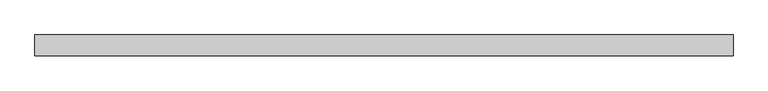
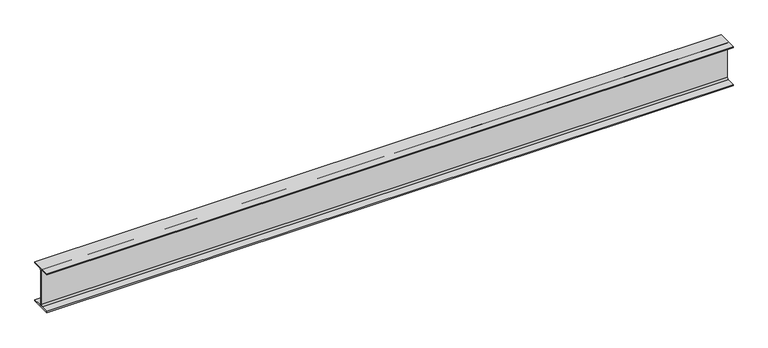
"""IFC4 building model written with IfcOpenShell, lengths in millimetres: beam geometry, 0912_Steel Framing_H-KSD3502 : H_SB_ASB_H-350x175x7x11."""

from ifc_helpers import new_model, si_unit, point, frame, frame_2d, origin, place, context, project, spatial, polyline, circle_curve, trimmed, segment, composite_curve, outline, extrude, source, transform, mapped, element, save


def beam_dbd466da(model_context):
    return source(origin(), model_context, "Body", "SweptSolid", [
        extrude(outline(composite_curve([segment(polyline([(87.5, -164.0), (87.5, -175.0), (-87.5, -175.0), (-87.5, -164.0), (-17.5, -164.0)]), True, "CONTINUOUS"), segment(trimmed(circle_curve(frame_2d((-17.5, -150.0)), 14.0), [point((-17.5, -164.0))], [point((-3.5, -150.0))], True, "CARTESIAN"), True, "CONTINUOUS"), segment(polyline([(-3.5, -150.0), (-3.5, 150.0)]), True, "CONTINUOUS"), segment(trimmed(circle_curve(frame_2d((-17.5, 150.0)), 14.0), [point((-3.5, 150.0))], [point((-17.5, 164.0))], True, "CARTESIAN"), True, "CONTINUOUS"), segment(polyline([(-17.5, 164.0), (-87.5, 164.0), (-87.5, 175.0), (87.5, 175.0), (87.5, 164.0), (17.5, 164.0)]), True, "CONTINUOUS"), segment(trimmed(circle_curve(frame_2d((17.5, 150.0)), 14.0), [point((17.5, 164.0))], [point((3.5, 150.0))], True, "CARTESIAN"), True, "CONTINUOUS"), segment(polyline([(3.5, 150.0), (3.5, -150.0)]), True, "CONTINUOUS"), segment(trimmed(circle_curve(frame_2d((17.5, -150.0)), 14.0), [point((3.5, -150.0))], [point((17.5, -164.0))], True, "CARTESIAN"), True, "CONTINUOUS"), segment(polyline([(17.5, -164.0), (87.5, -164.0)]), True, "CONTINUOUS")], self_intersect=False)), frame((-2912.1972294, 0.0, 0.0), z_axis=(1.0, 0.0, 0.0), x_axis=(0.0, 1.0, 0.0)), (0.0, 0.0, 1.0), 5810.2298939),
    ])


if __name__ == "__main__":
    model = new_model("IFC4")
    model_context = context("Model", 3, world=origin())
    ifc_project = project(units=[si_unit("LENGTHUNIT", "METRE", prefix="MILLI")], contexts=[model_context])
    site = spatial("IfcSite", under=ifc_project)
    building = spatial("IfcBuilding", under=site)
    placement = place(None, origin())
    beam_shape = beam_dbd466da(model_context)
    element("IfcBeam", 1, ObjectType="0912_Steel Framing_H-KSD3502 : H_SB_ASB_H-350x175x7x11", at=placement, inside=building, context=model_context, shape_type="MappedRepresentation", body=[
        mapped(beam_shape, transform((0.0, 0.0, 0.0), x_axis=(1.0, 0.0, 0.0), y_axis=(0.0, 1.0, 0.0), z_axis=(0.0, 0.0, 1.0))),
    ])
    save(model, "model.ifc")

# Revit data of these elements
# Type "0912_Steel Framing_H-KSD3502 : H_SB_ASB_H-350x175x7x11"
#   H_WM Code_1 = "S01AA002-00001 | Main Steel Structure Fabrication Work | Shelter/Building | Medium Steel - Standard (90KG/M>Weight≥30KG/M) | Material: (   )"
#   H_WM Code_2 = "S03AA028-00001 | Main Steel Structure Erection Work | Shelter/Building | Medium Steel (90KG/M>Weight≥30KG/M) | Material: (   )"
#   H_WM Code_3 = "S01AA010-00001 | Main Steel Structure Fabrication Work | Shelter/Building | Steel Painting/Coating | for Non-Fireproofed Steel Surface, Surface Preparation, Primer, Second & Final Coat | Material: (   )"
#   H_Q'ty Cal Type Tag = "SB-Q2"
#   Width = 17.5 cm
#   Web Thickness = 0.7 cm
#   Web Fillet = 1.4 cm
#   Warping Constant = 282000.0 cm⁶
#   W = 0
#   Torsional Moment of Inertia = 19.4042 cm⁴
#   Section Area = 63.14 cm²
#   Plastic Modulus weak axis = 174.0 cm³
#   Plastic Modulus strong axis = 868.0 cm³
#   Perimeter = 1.36 m²/m
#   Nominal Weight = 49.60 kgf/m
#   Moment of Inertia weak axis = 984.00 cm⁴
#   Moment of Inertia strong axis = 13600.00 cm⁴
#   Height = 35.0 cm
#   Flange Thickness = 1.1 cm
#   Elastic Modulus weak axis = 112.0 cm³
#   Elastic Modulus strong axis = 775.0 cm³
#   Centroid Vertical = 17.5 cm
#   Centroid Horizontal = 8.75 cm
#   Ix = 136000000
#   Length [instance default] = 1.5240 m
#   Zx = 868000
#   b = 0.1750 m
#   h = 0.3500 m
#   r = 0.0140 m
#   s = 0.0070 m
#   t = 0.0110 m
#   A = 0.006314 m²
#   Structural Material [instance default] = Steel, 45-345
#   Assembly Code = ""
# Element 1 (IfcBeam, "0912_Steel Framing_H-KSD3502 : H_SB_ASB_H-350x175x7x11")
#   Structural Material = none
# Materials
#   "Steel, 45-345": class "Metal", colour RGB 189 187 185, transparency 0, Description = "Steel 345 MPa", Cost = 0
